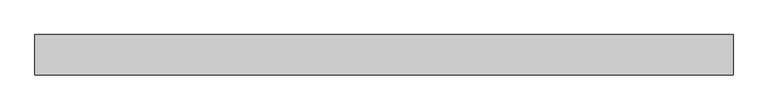
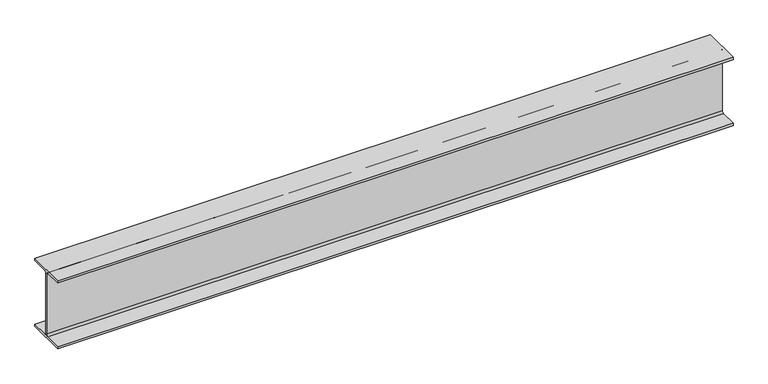
"""IFC4 building model written with IfcOpenShell, lengths in millimetres: beam geometry, Old_Steel Beam_H-KSD3502 : H_SB_ASB_H-200×200x8x12."""

from ifc_helpers import new_model, si_unit, point, frame, frame_2d, origin, place, context, project, spatial, polyline, circle_curve, trimmed, segment, composite_curve, outline, extrude, source, transform, mapped, element, save


def beam_3c3625a8(model_context):
    return source(origin(), model_context, "Body", "SweptSolid", [
        extrude(outline(composite_curve([segment(polyline([(82.5, -141.5), (82.5, -151.7), (-82.5, -151.7), (-82.5, -141.5), (-11.9, -141.5)]), True, "CONTINUOUS"), segment(trimmed(circle_curve(frame_2d((-11.9, -132.6)), 8.9), [point((-11.9, -141.5))], [point((-3.0, -132.6))], True, "CARTESIAN"), True, "CONTINUOUS"), segment(polyline([(-3.0, -132.6), (-3.0, 132.6)]), True, "CONTINUOUS"), segment(trimmed(circle_curve(frame_2d((-11.9, 132.6)), 8.9), [point((-3.0, 132.6))], [point((-11.9, 141.5))], True, "CARTESIAN"), True, "CONTINUOUS"), segment(polyline([(-11.9, 141.5), (-82.5, 141.5), (-82.5, 151.7), (82.5, 151.7), (82.5, 141.5), (11.9, 141.5)]), True, "CONTINUOUS"), segment(trimmed(circle_curve(frame_2d((11.9, 132.6)), 8.9), [point((11.9, 141.5))], [point((3.0, 132.6))], True, "CARTESIAN"), True, "CONTINUOUS"), segment(polyline([(3.0, 132.6), (3.0, -132.6)]), True, "CONTINUOUS"), segment(trimmed(circle_curve(frame_2d((11.9, -132.6)), 8.9), [point((3.0, -132.6))], [point((11.9, -141.5))], True, "CARTESIAN"), True, "CONTINUOUS"), segment(polyline([(11.9, -141.5), (82.5, -141.5)]), True, "CONTINUOUS")], self_intersect=False)), frame((-1255.552387, 0.0, 0.0), z_axis=(1.0, 0.0, 0.0), x_axis=(0.0, 1.0, 0.0)), (0.0, 0.0, 1.0), 2840.028729),
    ])


if __name__ == "__main__":
    model = new_model("IFC4")
    model_context = context("Model", 3, world=origin())
    ifc_project = project(units=[si_unit("LENGTHUNIT", "METRE", prefix="MILLI")], contexts=[model_context])
    site = spatial("IfcSite", under=ifc_project)
    building = spatial("IfcBuilding", under=site)
    placement = place(None, origin())
    beam_shape = beam_3c3625a8(model_context)
    element("IfcBeam", 1, ObjectType="Old_Steel Beam_H-KSD3502 : H_SB_ASB_H-200×200x8x12", at=placement, inside=building, context=model_context, shape_type="MappedRepresentation", body=[
        mapped(beam_shape, transform((0.0, 0.0, 0.0), x_axis=(1.0, 0.0, 0.0), y_axis=(0.0, 1.0, 0.0), z_axis=(0.0, 0.0, 1.0))),
    ])
    save(model, "model.ifc")

# Revit data of these elements
# Type "Old_Steel Beam_H-KSD3502 : H_SB_ASB_H-200×200x8x12"
#   Width = 20.0 cm
#   Web Thickness = 0.8 cm
#   Web Fillet = 1.3 cm
#   Warping Constant = 141376.0 cm⁶
#   Torsional Moment of Inertia = 26.2485 cm⁴
#   Torsional Modulus = 1.0 cm³
#   Section Area = 63.53 cm²
#   Plastic Modulus weak axis = 244.0 cm³
#   Plastic Modulus strong axis = 525.0 cm³
#   Perimeter = 1.16 m²/m
#   Nominal Weight = 49.90 kgf/m
#   Moment of Inertia weak axis = 1600.00 cm⁴
#   Moment of Inertia strong axis = 4720.00 cm⁴
#   Height = 20.0 cm
#   Flange Thickness = 1.2 cm
#   Elastic Modulus weak axis = 160.0 cm³
#   Elastic Modulus strong axis = 472.0 cm³
#   Centroid Vertical = 10.0 cm
#   Centroid Horizontal = 10.0 cm
#   Length [instance default] = 1.5240 m
#   Structural Material [instance default] = Steel, 45-345
#   Assembly Code = ""
# Element 1 (IfcBeam, "Old_Steel Beam_H-KSD3502 : H_SB_ASB_H-200×200x8x12")
#   Structural Material = none
# Materials
#   "Steel, 45-345": class "Metal", colour RGB 189 187 185, transparency 0, Description = "Steel 345 MPa", Cost = 0
